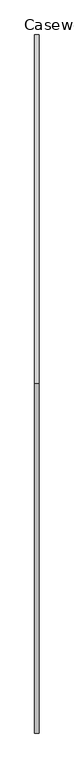
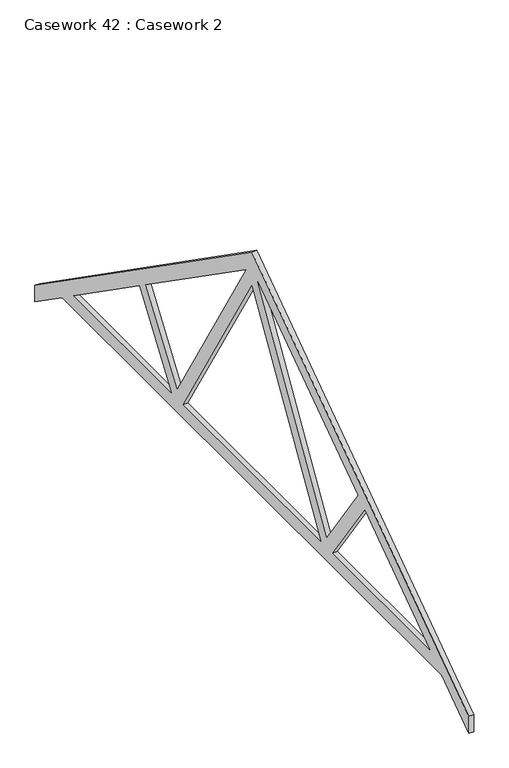
"""IFC4 building model written with IfcOpenShell, lengths in millimetres: furniture geometry, Casework 42 : Casework 2."""

import ifcopenshell
import ifcopenshell.guid

model = None  # the IFC model being written
_history = None  # IfcOwnerHistory: only IFC2X3 demands one
_inside = {}  # id of a spatial element -> (the spatial element, [elements in it])
_under = {}  # id of a project, library or spatial element -> (it, [spatial elements below it])
_declared = {}  # id of a project -> (the project, [libraries it declares])
_typed = {}  # id of a type object -> (the type object, [elements of that type])
_made_of = {}  # id of a material, layer set ... -> (it, [elements and type objects made of it])


def new_model(schema):
    """Start an empty IFC model of exactly this schema.

    Asked for "IFC4X3", IfcOpenShell would pick the latest addendum, in which some entities
    have other attributes; the version numbers below select the first issue.
    IFC2X3 requires an IfcOwnerHistory on every rooted entity: one is made here for all.
    """
    global model, _history
    if schema == "IFC4X3":
        model = ifcopenshell.file(schema_version=(4, 3, 0, 0))
    else:
        model = ifcopenshell.file(schema=schema)
    _inside.clear()
    _under.clear()
    _declared.clear()
    _typed.clear()
    _made_of.clear()
    _history = None
    if model.schema == "IFC2X3":
        org = make("IfcOrganization", Name="unknown")
        user = make(
            "IfcPersonAndOrganization",
            ThePerson=make("IfcPerson", FamilyName="unknown"),
            TheOrganization=org,
        )
        app = make(
            "IfcApplication",
            ApplicationDeveloper=org,
            Version="unknown",
            ApplicationFullName="unknown",
            ApplicationIdentifier="unknown",
        )
        _history = make(
            "IfcOwnerHistory",
            OwningUser=user,
            OwningApplication=app,
            ChangeAction="ADDED",
            CreationDate=0,
        )
    return model


def make(cls, **values):
    """One entity of the class cls with the attributes given. An attribute that is None is left unset."""
    return model.create_entity(
        cls, **{name: value for name, value in values.items() if value is not None}
    )


def rooted(cls, **values):
    """An entity with a GlobalId (a new one), such as an element, a storey or a relation."""
    return make(cls, GlobalId=ifcopenshell.guid.new(), OwnerHistory=_history, **values)


def si_unit(unit_type, name, prefix=None):
    """IfcSIUnit, for example si_unit("LENGTHUNIT", "METRE", prefix="MILLI")."""
    return make("IfcSIUnit", UnitType=unit_type, Prefix=prefix, Name=name)


def assignment(units):
    """IfcUnitAssignment: the units of a project."""
    return None if units is None else make("IfcUnitAssignment", Units=units)


def point(xyz):
    """IfcCartesianPoint."""
    return None if xyz is None else make("IfcCartesianPoint", Coordinates=xyz)


def direction(xyz):
    """IfcDirection."""
    return None if xyz is None else make("IfcDirection", DirectionRatios=xyz)


def frame(location, z_axis=None, x_axis=None):
    """IfcAxis2Placement3D, a coordinate frame: its origin and axes. An axis left out is left unset."""
    return make(
        "IfcAxis2Placement3D",
        Location=point(location),
        Axis=direction(z_axis),
        RefDirection=direction(x_axis),
    )


def origin():
    """The frame at (0, 0, 0) with its axes left unset."""
    return frame((0.0, 0.0, 0.0))


def place(relative_to, where):
    """IfcLocalPlacement: puts the frame where relative to a parent placement (None: the world)."""
    return make(
        "IfcLocalPlacement", PlacementRelTo=relative_to, RelativePlacement=where
    )


def context(
    kind, dimensions, precision=None, world=None, true_north=None, identifier=None
):
    """IfcGeometricRepresentationContext, for example the 3D "Model" context."""
    return make(
        "IfcGeometricRepresentationContext",
        ContextIdentifier=identifier,
        ContextType=kind,
        CoordinateSpaceDimension=dimensions,
        Precision=precision,
        WorldCoordinateSystem=world,
        TrueNorth=true_north,
    )


def project(units=None, contexts=None):
    """IfcProject with its units and contexts."""
    return rooted(
        "IfcProject",
        Name="project",
        RepresentationContexts=contexts,
        UnitsInContext=assignment(units),
    )


def spatial(cls, under=None, at=None, **own):
    """A site, building, storey or space (cls), placed at a placement, below another one or the project."""
    s = rooted(cls, ObjectPlacement=at, **own)
    if under is not None:
        _under.setdefault(under.id(), (under, []))[1].append(s)
    return s


def polyline(points):
    """IfcPolyline through the points."""
    return make("IfcPolyline", Points=[point(p) for p in points])


def outline(outer, holes=None, kind="AREA"):
    """IfcArbitraryClosedProfileDef: a profile drawn as a closed curve; with holes, ...WithVoids."""
    if holes is None:
        return make("IfcArbitraryClosedProfileDef", ProfileType=kind, OuterCurve=outer)
    return make(
        "IfcArbitraryProfileDefWithVoids",
        ProfileType=kind,
        OuterCurve=outer,
        InnerCurves=holes,
    )


def extrude(swept, where, along, depth):
    """IfcExtrudedAreaSolid: the profile swept, set in the frame where, extruded along a direction by depth."""
    return make(
        "IfcExtrudedAreaSolid",
        SweptArea=swept,
        Position=where,
        ExtrudedDirection=direction(along),
        Depth=depth,
    )


def shape(context_of_items, identifier, shape_type, items):
    """IfcShapeRepresentation: the items that make up one representation, for example the "Body"."""
    return make(
        "IfcShapeRepresentation",
        ContextOfItems=context_of_items,
        RepresentationIdentifier=identifier,
        RepresentationType=shape_type,
        Items=items,
    )


def source(mapping_origin, context_of_items, identifier, shape_type, items):
    """IfcRepresentationMap: a shape defined once, which mapped items show again and again."""
    return make(
        "IfcRepresentationMap",
        MappingOrigin=mapping_origin,
        MappedRepresentation=shape(context_of_items, identifier, shape_type, items),
    )


def transform(
    local_origin,
    x_axis=None,
    y_axis=None,
    z_axis=None,
    scale=None,
    scale2=None,
    scale3=None,
    uniform=True,
):
    """IfcCartesianTransformationOperator3D, or its non-uniform kind. x_axis, y_axis, z_axis: its Axis1, 2, 3."""
    if uniform:
        return make(
            "IfcCartesianTransformationOperator3D",
            Axis1=direction(x_axis),
            Axis2=direction(y_axis),
            LocalOrigin=point(local_origin),
            Scale=scale,
            Axis3=direction(z_axis),
        )
    return make(
        "IfcCartesianTransformationOperator3DnonUniform",
        Axis1=direction(x_axis),
        Axis2=direction(y_axis),
        LocalOrigin=point(local_origin),
        Scale=scale,
        Axis3=direction(z_axis),
        Scale2=scale2,
        Scale3=scale3,
    )


def mapped(mapping_source, mapping_target):
    """IfcMappedItem: shows the shape of a source again, moved by a transform."""
    return make(
        "IfcMappedItem", MappingSource=mapping_source, MappingTarget=mapping_target
    )


def made_of(thing, what):
    """Note that an element or type object is made of a material, layer set ...; save() writes the relation."""
    if what is not None:
        _made_of.setdefault(what.id(), (what, []))[1].append(thing)
    return thing


def element(
    cls,
    number,
    at=None,
    inside=None,
    cuts=None,
    type_object=None,
    material=None,
    context=None,
    identifier="Body",
    shape_type=None,
    held_by="IfcProductDefinitionShape",
    body=None,
    shapes=None,
    **own,
):
    """One element of the class cls, such as IfcWall. Its Tag is "e" and its number.

    at: its placement. inside: the storey or other place that contains it. cuts: it is an
    opening in that element (IfcRelVoidsElement). A single representation is given by context,
    identifier, shape_type and body (its items); several are given by shapes. held_by: the class
    of the entity that holds the representations. save() writes the other relations.
    """
    e = rooted(cls, Tag="e%d" % number, ObjectPlacement=at, **own)
    if body is not None:
        shapes = [shape(context, identifier, shape_type, body)]
    if shapes is not None:
        e.Representation = make(held_by, Representations=shapes)
    if inside is not None:
        _inside.setdefault(inside.id(), (inside, []))[1].append(e)
    if cuts is not None:
        rooted(
            "IfcRelVoidsElement", RelatingBuildingElement=cuts, RelatedOpeningElement=e
        )
    if type_object is not None:
        _typed.setdefault(type_object.id(), (type_object, []))[1].append(e)
    return made_of(e, material)


def aggregate(whole, parts):
    """IfcRelAggregates: a whole, such as a stair, and the parts it consists of."""
    return rooted("IfcRelAggregates", RelatingObject=whole, RelatedObjects=parts)


def save(model, path):
    """Write the relations noted so far, then the file.

    IfcRelAggregates (storeys below a building ...), IfcRelContainedInSpatialStructure (elements
    in a storey), IfcRelDefinesByType, IfcRelAssociatesMaterial and IfcRelDeclares: one each for
    every whole, place, type object, material and project.
    """
    for whole, parts in _under.values():
        aggregate(whole, parts)
    for where, things in _inside.values():
        rooted(
            "IfcRelContainedInSpatialStructure",
            RelatedElements=things,
            RelatingStructure=where,
        )
    for kind, things in _typed.values():
        rooted("IfcRelDefinesByType", RelatedObjects=things, RelatingType=kind)
    for what, things in _made_of.values():
        rooted("IfcRelAssociatesMaterial", RelatedObjects=things, RelatingMaterial=what)
    for by, libraries in _declared.values():
        rooted("IfcRelDeclares", RelatingContext=by, RelatedDefinitions=libraries)
    model.write(path)


def casework_42_casework_2_e9decabd(model_context):
    return source(origin(), model_context, "Body", "SweptSolid", [
        extrude(outline(polyline([(6583.1149316, 5252.5), (-277.3850684, 5252.5), (-767.3850684, 4909.3983063), (-767.3850684, 5092.5144946), (3152.8649316, 7837.5030963), (7073.1149316, 5092.5144946), (7073.1149316, 4909.3983063), (6583.1149316, 5252.5)]), holes=[polyline([(4612.3149663, 5402.5), (6368.8927306, 5402.5), (5190.2113591, 6227.8215815), (4612.3149663, 5402.5)]), polyline([(4394.2037684, 5402.5), (3152.8649316, 7468.4347567), (1911.5260948, 5402.5), (4394.2037684, 5402.5)]), polyline([(4504.5438357, 5510.1038939), (5067.3385525, 6313.8580469), (3262.0771677, 7577.915677), (4504.5438357, 5510.1038939)]), polyline([(1693.4148969, 5402.5), (1115.5185041, 6227.8215815), (-63.1628674, 5402.5), (1693.4148969, 5402.5)]), polyline([(1801.1860276, 5510.1038939), (3043.6526956, 7577.915677), (1238.3913108, 6313.8580469), (1801.1860276, 5510.1038939)])]), frame((-8021.5247381, 0.0, 0.0), z_axis=(1.0, 0.0, 0.0), x_axis=(0.0, 1.0, 0.0)), (0.0, 0.0, 1.0), 49.6351915),
    ])


if __name__ == "__main__":
    model = new_model("IFC4")
    model_context = context("Model", 3, world=origin())
    ifc_project = project(units=[si_unit("LENGTHUNIT", "METRE", prefix="MILLI")], contexts=[model_context])
    site = spatial("IfcSite", under=ifc_project)
    building = spatial("IfcBuilding", under=site)
    placement = place(None, origin())
    casework_42_casework_2_shape = casework_42_casework_2_e9decabd(model_context)
    element("IfcFurniture", 1, ObjectType="Casework 42 : Casework 2", at=placement, inside=building, context=model_context, shape_type="MappedRepresentation", body=[
        mapped(casework_42_casework_2_shape, transform((0.0, 0.0, 0.0), x_axis=(1.0, 0.0, 0.0), y_axis=(0.0, 1.0, 0.0), z_axis=(0.0, 0.0, 1.0))),
    ])
    save(model, "model.ifc")

# Revit data of these elements
# Element 1 (IfcFurniture, "Casework 42 : Casework 2")
#   Materials on its faces: "Softwood, Lumber"
# Materials
#   "Softwood, Lumber": class "Wood", colour RGB 205 156 65, transparency 0, Description = "Pinus Echinata", Cost = 0
